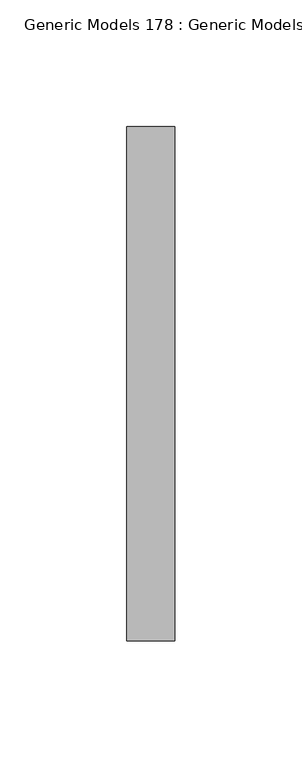
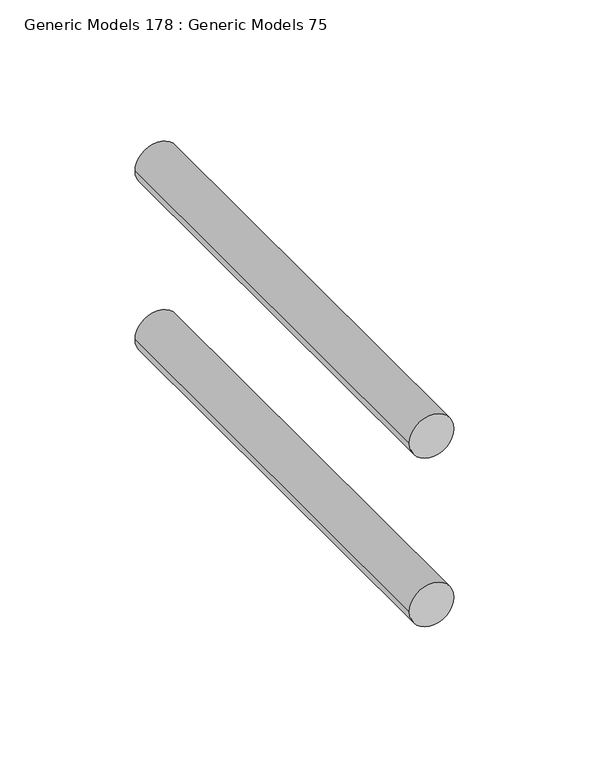
"""IFC4 building model written with IfcOpenShell, lengths in millimetres: proxy geometry, Generic Models 178 : Generic Models 75."""

import ifcopenshell
import ifcopenshell.guid

model = None  # the IFC model being written
_history = None  # IfcOwnerHistory: only IFC2X3 demands one
_inside = {}  # id of a spatial element -> (the spatial element, [elements in it])
_under = {}  # id of a project, library or spatial element -> (it, [spatial elements below it])
_declared = {}  # id of a project -> (the project, [libraries it declares])
_typed = {}  # id of a type object -> (the type object, [elements of that type])
_made_of = {}  # id of a material, layer set ... -> (it, [elements and type objects made of it])


def new_model(schema):
    """Start an empty IFC model of exactly this schema.

    Asked for "IFC4X3", IfcOpenShell would pick the latest addendum, in which some entities
    have other attributes; the version numbers below select the first issue.
    IFC2X3 requires an IfcOwnerHistory on every rooted entity: one is made here for all.
    """
    global model, _history
    if schema == "IFC4X3":
        model = ifcopenshell.file(schema_version=(4, 3, 0, 0))
    else:
        model = ifcopenshell.file(schema=schema)
    _inside.clear()
    _under.clear()
    _declared.clear()
    _typed.clear()
    _made_of.clear()
    _history = None
    if model.schema == "IFC2X3":
        org = make("IfcOrganization", Name="unknown")
        user = make(
            "IfcPersonAndOrganization",
            ThePerson=make("IfcPerson", FamilyName="unknown"),
            TheOrganization=org,
        )
        app = make(
            "IfcApplication",
            ApplicationDeveloper=org,
            Version="unknown",
            ApplicationFullName="unknown",
            ApplicationIdentifier="unknown",
        )
        _history = make(
            "IfcOwnerHistory",
            OwningUser=user,
            OwningApplication=app,
            ChangeAction="ADDED",
            CreationDate=0,
        )
    return model


def make(cls, **values):
    """One entity of the class cls with the attributes given. An attribute that is None is left unset."""
    return model.create_entity(
        cls, **{name: value for name, value in values.items() if value is not None}
    )


def rooted(cls, **values):
    """An entity with a GlobalId (a new one), such as an element, a storey or a relation."""
    return make(cls, GlobalId=ifcopenshell.guid.new(), OwnerHistory=_history, **values)


def si_unit(unit_type, name, prefix=None):
    """IfcSIUnit, for example si_unit("LENGTHUNIT", "METRE", prefix="MILLI")."""
    return make("IfcSIUnit", UnitType=unit_type, Prefix=prefix, Name=name)


def assignment(units):
    """IfcUnitAssignment: the units of a project."""
    return None if units is None else make("IfcUnitAssignment", Units=units)


def point(xyz):
    """IfcCartesianPoint."""
    return None if xyz is None else make("IfcCartesianPoint", Coordinates=xyz)


def direction(xyz):
    """IfcDirection."""
    return None if xyz is None else make("IfcDirection", DirectionRatios=xyz)


def frame(location, z_axis=None, x_axis=None):
    """IfcAxis2Placement3D, a coordinate frame: its origin and axes. An axis left out is left unset."""
    return make(
        "IfcAxis2Placement3D",
        Location=point(location),
        Axis=direction(z_axis),
        RefDirection=direction(x_axis),
    )


def frame_2d(location, x_axis=None):
    """IfcAxis2Placement2D, a coordinate frame in the plane: its origin and x axis."""
    return make(
        "IfcAxis2Placement2D", Location=point(location), RefDirection=direction(x_axis)
    )


def origin():
    """The frame at (0, 0, 0) with its axes left unset."""
    return frame((0.0, 0.0, 0.0))


def place(relative_to, where):
    """IfcLocalPlacement: puts the frame where relative to a parent placement (None: the world)."""
    return make(
        "IfcLocalPlacement", PlacementRelTo=relative_to, RelativePlacement=where
    )


def context(
    kind, dimensions, precision=None, world=None, true_north=None, identifier=None
):
    """IfcGeometricRepresentationContext, for example the 3D "Model" context."""
    return make(
        "IfcGeometricRepresentationContext",
        ContextIdentifier=identifier,
        ContextType=kind,
        CoordinateSpaceDimension=dimensions,
        Precision=precision,
        WorldCoordinateSystem=world,
        TrueNorth=true_north,
    )


def project(units=None, contexts=None):
    """IfcProject with its units and contexts."""
    return rooted(
        "IfcProject",
        Name="project",
        RepresentationContexts=contexts,
        UnitsInContext=assignment(units),
    )


def spatial(cls, under=None, at=None, **own):
    """A site, building, storey or space (cls), placed at a placement, below another one or the project."""
    s = rooted(cls, ObjectPlacement=at, **own)
    if under is not None:
        _under.setdefault(under.id(), (under, []))[1].append(s)
    return s


def circle_curve(where, radius):
    """IfcCircle in the frame where."""
    return make("IfcCircle", Position=where, Radius=radius)


def trimmed(basis, trim1, trim2, sense, master):
    """IfcTrimmedCurve: the piece of a basis curve between two trims."""
    return make(
        "IfcTrimmedCurve",
        BasisCurve=basis,
        Trim1=trim1,
        Trim2=trim2,
        SenseAgreement=sense,
        MasterRepresentation=master,
    )


def segment(curve, same_sense, transition):
    """IfcCompositeCurveSegment."""
    return make(
        "IfcCompositeCurveSegment",
        Transition=transition,
        SameSense=same_sense,
        ParentCurve=curve,
    )


def composite_curve(segments, self_intersect=None):
    """IfcCompositeCurve: segments joined end to end."""
    return make("IfcCompositeCurve", Segments=segments, SelfIntersect=self_intersect)


def outline(outer, holes=None, kind="AREA"):
    """IfcArbitraryClosedProfileDef: a profile drawn as a closed curve; with holes, ...WithVoids."""
    if holes is None:
        return make("IfcArbitraryClosedProfileDef", ProfileType=kind, OuterCurve=outer)
    return make(
        "IfcArbitraryProfileDefWithVoids",
        ProfileType=kind,
        OuterCurve=outer,
        InnerCurves=holes,
    )


def extrude(swept, where, along, depth):
    """IfcExtrudedAreaSolid: the profile swept, set in the frame where, extruded along a direction by depth."""
    return make(
        "IfcExtrudedAreaSolid",
        SweptArea=swept,
        Position=where,
        ExtrudedDirection=direction(along),
        Depth=depth,
    )


def shape(context_of_items, identifier, shape_type, items):
    """IfcShapeRepresentation: the items that make up one representation, for example the "Body"."""
    return make(
        "IfcShapeRepresentation",
        ContextOfItems=context_of_items,
        RepresentationIdentifier=identifier,
        RepresentationType=shape_type,
        Items=items,
    )


def source(mapping_origin, context_of_items, identifier, shape_type, items):
    """IfcRepresentationMap: a shape defined once, which mapped items show again and again."""
    return make(
        "IfcRepresentationMap",
        MappingOrigin=mapping_origin,
        MappedRepresentation=shape(context_of_items, identifier, shape_type, items),
    )


def transform(
    local_origin,
    x_axis=None,
    y_axis=None,
    z_axis=None,
    scale=None,
    scale2=None,
    scale3=None,
    uniform=True,
):
    """IfcCartesianTransformationOperator3D, or its non-uniform kind. x_axis, y_axis, z_axis: its Axis1, 2, 3."""
    if uniform:
        return make(
            "IfcCartesianTransformationOperator3D",
            Axis1=direction(x_axis),
            Axis2=direction(y_axis),
            LocalOrigin=point(local_origin),
            Scale=scale,
            Axis3=direction(z_axis),
        )
    return make(
        "IfcCartesianTransformationOperator3DnonUniform",
        Axis1=direction(x_axis),
        Axis2=direction(y_axis),
        LocalOrigin=point(local_origin),
        Scale=scale,
        Axis3=direction(z_axis),
        Scale2=scale2,
        Scale3=scale3,
    )


def mapped(mapping_source, mapping_target):
    """IfcMappedItem: shows the shape of a source again, moved by a transform."""
    return make(
        "IfcMappedItem", MappingSource=mapping_source, MappingTarget=mapping_target
    )


def made_of(thing, what):
    """Note that an element or type object is made of a material, layer set ...; save() writes the relation."""
    if what is not None:
        _made_of.setdefault(what.id(), (what, []))[1].append(thing)
    return thing


def element(
    cls,
    number,
    at=None,
    inside=None,
    cuts=None,
    type_object=None,
    material=None,
    context=None,
    identifier="Body",
    shape_type=None,
    held_by="IfcProductDefinitionShape",
    body=None,
    shapes=None,
    **own,
):
    """One element of the class cls, such as IfcWall. Its Tag is "e" and its number.

    at: its placement. inside: the storey or other place that contains it. cuts: it is an
    opening in that element (IfcRelVoidsElement). A single representation is given by context,
    identifier, shape_type and body (its items); several are given by shapes. held_by: the class
    of the entity that holds the representations. save() writes the other relations.
    """
    e = rooted(cls, Tag="e%d" % number, ObjectPlacement=at, **own)
    if body is not None:
        shapes = [shape(context, identifier, shape_type, body)]
    if shapes is not None:
        e.Representation = make(held_by, Representations=shapes)
    if inside is not None:
        _inside.setdefault(inside.id(), (inside, []))[1].append(e)
    if cuts is not None:
        rooted(
            "IfcRelVoidsElement", RelatingBuildingElement=cuts, RelatedOpeningElement=e
        )
    if type_object is not None:
        _typed.setdefault(type_object.id(), (type_object, []))[1].append(e)
    return made_of(e, material)


def aggregate(whole, parts):
    """IfcRelAggregates: a whole, such as a stair, and the parts it consists of."""
    return rooted("IfcRelAggregates", RelatingObject=whole, RelatedObjects=parts)


def save(model, path):
    """Write the relations noted so far, then the file.

    IfcRelAggregates (storeys below a building ...), IfcRelContainedInSpatialStructure (elements
    in a storey), IfcRelDefinesByType, IfcRelAssociatesMaterial and IfcRelDeclares: one each for
    every whole, place, type object, material and project.
    """
    for whole, parts in _under.values():
        aggregate(whole, parts)
    for where, things in _inside.values():
        rooted(
            "IfcRelContainedInSpatialStructure",
            RelatedElements=things,
            RelatingStructure=where,
        )
    for kind, things in _typed.values():
        rooted("IfcRelDefinesByType", RelatedObjects=things, RelatingType=kind)
    for what, things in _made_of.values():
        rooted("IfcRelAssociatesMaterial", RelatedObjects=things, RelatingMaterial=what)
    for by, libraries in _declared.values():
        rooted("IfcRelDeclares", RelatingContext=by, RelatedDefinitions=libraries)
    model.write(path)


def generic_models_178_generic_models_75_fd17830b(model_context):
    return source(origin(), model_context, "Body", "SweptSolid", [
        extrude(outline(composite_curve([segment(trimmed(circle_curve(frame_2d((271765.7125, 31975.4096032)), 9.525), [point((271765.7125, 31965.8846032))], [point((271765.7125, 31984.9346032))], False, "CARTESIAN"), True, "CONTINUOUS"), segment(trimmed(circle_curve(frame_2d((271765.7125, 31975.4096032)), 9.525), [point((271765.7125, 31984.9346032))], [point((271765.7125, 31965.8846032))], False, "CARTESIAN"), True, "CONTINUOUS")], self_intersect=False)), frame((0.0, 36305.8207942, 0.0), z_axis=(0.0, 1.0, 0.0), x_axis=(0.0, 0.0, 1.0)), (0.0, 0.0, 1.0), 203.2),
        extrude(outline(composite_curve([segment(trimmed(circle_curve(frame_2d((271841.9125, 31975.4096032)), 9.525), [point((271841.9125, 31965.8846032))], [point((271841.9125, 31984.9346032))], False, "CARTESIAN"), True, "CONTINUOUS"), segment(trimmed(circle_curve(frame_2d((271841.9125, 31975.4096032)), 9.525), [point((271841.9125, 31984.9346032))], [point((271841.9125, 31965.8846032))], False, "CARTESIAN"), True, "CONTINUOUS")], self_intersect=False)), frame((0.0, 36305.8207942, 0.0), z_axis=(0.0, 1.0, 0.0), x_axis=(0.0, 0.0, 1.0)), (0.0, 0.0, 1.0), 203.2),
    ])


if __name__ == "__main__":
    model = new_model("IFC4")
    model_context = context("Model", 3, world=origin())
    ifc_project = project(units=[si_unit("LENGTHUNIT", "METRE", prefix="MILLI")], contexts=[model_context])
    site = spatial("IfcSite", under=ifc_project)
    building = spatial("IfcBuilding", under=site)
    placement = place(None, origin())
    generic_models_178_generic_models_75_shape = generic_models_178_generic_models_75_fd17830b(model_context)
    element("IfcBuildingElementProxy", 1, Name="Generic Models 178 : Generic Models 75", ObjectType="Generic Models 178 : Generic Models 75", at=placement, inside=building, context=model_context, shape_type="MappedRepresentation", body=[
        mapped(generic_models_178_generic_models_75_shape, transform((0.0, 0.0, 0.0), x_axis=(1.0, 0.0, 0.0), y_axis=(0.0, 1.0, 0.0), z_axis=(0.0, 0.0, 1.0))),
    ])
    save(model, "model.ifc")
